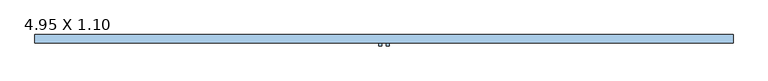
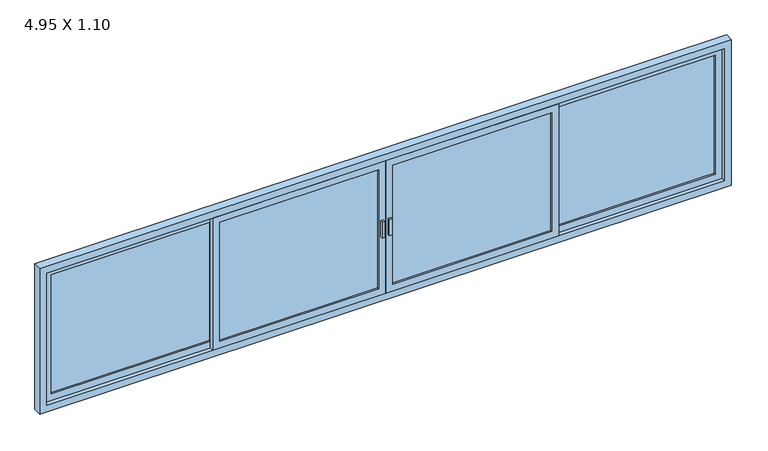
"""IFC4 building model written with IfcOpenShell, lengths in millimetres: window geometry, .CC_ND 300_JANELA_4 FOLHAS DE CORRER_VIDRO : 4.95 X 1.10."""

import ifcopenshell
import ifcopenshell.guid

model = None  # the IFC model being written
_history = None  # IfcOwnerHistory: only IFC2X3 demands one
_inside = {}  # id of a spatial element -> (the spatial element, [elements in it])
_under = {}  # id of a project, library or spatial element -> (it, [spatial elements below it])
_declared = {}  # id of a project -> (the project, [libraries it declares])
_typed = {}  # id of a type object -> (the type object, [elements of that type])
_made_of = {}  # id of a material, layer set ... -> (it, [elements and type objects made of it])


def new_model(schema):
    """Start an empty IFC model of exactly this schema.

    Asked for "IFC4X3", IfcOpenShell would pick the latest addendum, in which some entities
    have other attributes; the version numbers below select the first issue.
    IFC2X3 requires an IfcOwnerHistory on every rooted entity: one is made here for all.
    """
    global model, _history
    if schema == "IFC4X3":
        model = ifcopenshell.file(schema_version=(4, 3, 0, 0))
    else:
        model = ifcopenshell.file(schema=schema)
    _inside.clear()
    _under.clear()
    _declared.clear()
    _typed.clear()
    _made_of.clear()
    _history = None
    if model.schema == "IFC2X3":
        org = make("IfcOrganization", Name="unknown")
        user = make(
            "IfcPersonAndOrganization",
            ThePerson=make("IfcPerson", FamilyName="unknown"),
            TheOrganization=org,
        )
        app = make(
            "IfcApplication",
            ApplicationDeveloper=org,
            Version="unknown",
            ApplicationFullName="unknown",
            ApplicationIdentifier="unknown",
        )
        _history = make(
            "IfcOwnerHistory",
            OwningUser=user,
            OwningApplication=app,
            ChangeAction="ADDED",
            CreationDate=0,
        )
    return model


def make(cls, **values):
    """One entity of the class cls with the attributes given. An attribute that is None is left unset."""
    return model.create_entity(
        cls, **{name: value for name, value in values.items() if value is not None}
    )


def rooted(cls, **values):
    """An entity with a GlobalId (a new one), such as an element, a storey or a relation."""
    return make(cls, GlobalId=ifcopenshell.guid.new(), OwnerHistory=_history, **values)


def si_unit(unit_type, name, prefix=None):
    """IfcSIUnit, for example si_unit("LENGTHUNIT", "METRE", prefix="MILLI")."""
    return make("IfcSIUnit", UnitType=unit_type, Prefix=prefix, Name=name)


def assignment(units):
    """IfcUnitAssignment: the units of a project."""
    return None if units is None else make("IfcUnitAssignment", Units=units)


def point(xyz):
    """IfcCartesianPoint."""
    return None if xyz is None else make("IfcCartesianPoint", Coordinates=xyz)


def direction(xyz):
    """IfcDirection."""
    return None if xyz is None else make("IfcDirection", DirectionRatios=xyz)


def frame(location, z_axis=None, x_axis=None):
    """IfcAxis2Placement3D, a coordinate frame: its origin and axes. An axis left out is left unset."""
    return make(
        "IfcAxis2Placement3D",
        Location=point(location),
        Axis=direction(z_axis),
        RefDirection=direction(x_axis),
    )


def origin():
    """The frame at (0, 0, 0) with its axes left unset."""
    return frame((0.0, 0.0, 0.0))


def place(relative_to, where):
    """IfcLocalPlacement: puts the frame where relative to a parent placement (None: the world)."""
    return make(
        "IfcLocalPlacement", PlacementRelTo=relative_to, RelativePlacement=where
    )


def context(
    kind, dimensions, precision=None, world=None, true_north=None, identifier=None
):
    """IfcGeometricRepresentationContext, for example the 3D "Model" context."""
    return make(
        "IfcGeometricRepresentationContext",
        ContextIdentifier=identifier,
        ContextType=kind,
        CoordinateSpaceDimension=dimensions,
        Precision=precision,
        WorldCoordinateSystem=world,
        TrueNorth=true_north,
    )


def project(units=None, contexts=None):
    """IfcProject with its units and contexts."""
    return rooted(
        "IfcProject",
        Name="project",
        RepresentationContexts=contexts,
        UnitsInContext=assignment(units),
    )


def spatial(cls, under=None, at=None, **own):
    """A site, building, storey or space (cls), placed at a placement, below another one or the project."""
    s = rooted(cls, ObjectPlacement=at, **own)
    if under is not None:
        _under.setdefault(under.id(), (under, []))[1].append(s)
    return s


def polyline(points):
    """IfcPolyline through the points."""
    return make("IfcPolyline", Points=[point(p) for p in points])


def outline(outer, holes=None, kind="AREA"):
    """IfcArbitraryClosedProfileDef: a profile drawn as a closed curve; with holes, ...WithVoids."""
    if holes is None:
        return make("IfcArbitraryClosedProfileDef", ProfileType=kind, OuterCurve=outer)
    return make(
        "IfcArbitraryProfileDefWithVoids",
        ProfileType=kind,
        OuterCurve=outer,
        InnerCurves=holes,
    )


def extrude(swept, where, along, depth):
    """IfcExtrudedAreaSolid: the profile swept, set in the frame where, extruded along a direction by depth."""
    return make(
        "IfcExtrudedAreaSolid",
        SweptArea=swept,
        Position=where,
        ExtrudedDirection=direction(along),
        Depth=depth,
    )


def shape(context_of_items, identifier, shape_type, items):
    """IfcShapeRepresentation: the items that make up one representation, for example the "Body"."""
    return make(
        "IfcShapeRepresentation",
        ContextOfItems=context_of_items,
        RepresentationIdentifier=identifier,
        RepresentationType=shape_type,
        Items=items,
    )


def source(mapping_origin, context_of_items, identifier, shape_type, items):
    """IfcRepresentationMap: a shape defined once, which mapped items show again and again."""
    return make(
        "IfcRepresentationMap",
        MappingOrigin=mapping_origin,
        MappedRepresentation=shape(context_of_items, identifier, shape_type, items),
    )


def transform(
    local_origin,
    x_axis=None,
    y_axis=None,
    z_axis=None,
    scale=None,
    scale2=None,
    scale3=None,
    uniform=True,
):
    """IfcCartesianTransformationOperator3D, or its non-uniform kind. x_axis, y_axis, z_axis: its Axis1, 2, 3."""
    if uniform:
        return make(
            "IfcCartesianTransformationOperator3D",
            Axis1=direction(x_axis),
            Axis2=direction(y_axis),
            LocalOrigin=point(local_origin),
            Scale=scale,
            Axis3=direction(z_axis),
        )
    return make(
        "IfcCartesianTransformationOperator3DnonUniform",
        Axis1=direction(x_axis),
        Axis2=direction(y_axis),
        LocalOrigin=point(local_origin),
        Scale=scale,
        Axis3=direction(z_axis),
        Scale2=scale2,
        Scale3=scale3,
    )


def mapped(mapping_source, mapping_target):
    """IfcMappedItem: shows the shape of a source again, moved by a transform."""
    return make(
        "IfcMappedItem", MappingSource=mapping_source, MappingTarget=mapping_target
    )


def made_of(thing, what):
    """Note that an element or type object is made of a material, layer set ...; save() writes the relation."""
    if what is not None:
        _made_of.setdefault(what.id(), (what, []))[1].append(thing)
    return thing


def element(
    cls,
    number,
    at=None,
    inside=None,
    cuts=None,
    type_object=None,
    material=None,
    context=None,
    identifier="Body",
    shape_type=None,
    held_by="IfcProductDefinitionShape",
    body=None,
    shapes=None,
    **own,
):
    """One element of the class cls, such as IfcWall. Its Tag is "e" and its number.

    at: its placement. inside: the storey or other place that contains it. cuts: it is an
    opening in that element (IfcRelVoidsElement). A single representation is given by context,
    identifier, shape_type and body (its items); several are given by shapes. held_by: the class
    of the entity that holds the representations. save() writes the other relations.
    """
    e = rooted(cls, Tag="e%d" % number, ObjectPlacement=at, **own)
    if body is not None:
        shapes = [shape(context, identifier, shape_type, body)]
    if shapes is not None:
        e.Representation = make(held_by, Representations=shapes)
    if inside is not None:
        _inside.setdefault(inside.id(), (inside, []))[1].append(e)
    if cuts is not None:
        rooted(
            "IfcRelVoidsElement", RelatingBuildingElement=cuts, RelatedOpeningElement=e
        )
    if type_object is not None:
        _typed.setdefault(type_object.id(), (type_object, []))[1].append(e)
    return made_of(e, material)


def aggregate(whole, parts):
    """IfcRelAggregates: a whole, such as a stair, and the parts it consists of."""
    return rooted("IfcRelAggregates", RelatingObject=whole, RelatedObjects=parts)


def save(model, path):
    """Write the relations noted so far, then the file.

    IfcRelAggregates (storeys below a building ...), IfcRelContainedInSpatialStructure (elements
    in a storey), IfcRelDefinesByType, IfcRelAssociatesMaterial and IfcRelDeclares: one each for
    every whole, place, type object, material and project.
    """
    for whole, parts in _under.values():
        aggregate(whole, parts)
    for where, things in _inside.values():
        rooted(
            "IfcRelContainedInSpatialStructure",
            RelatedElements=things,
            RelatingStructure=where,
        )
    for kind, things in _typed.values():
        rooted("IfcRelDefinesByType", RelatedObjects=things, RelatingType=kind)
    for what, things in _made_of.values():
        rooted("IfcRelAssociatesMaterial", RelatedObjects=things, RelatingMaterial=what)
    for by, libraries in _declared.values():
        rooted("IfcRelDeclares", RelatingContext=by, RelatedDefinitions=libraries)
    model.write(path)


def window_4_95_x_1_10_4a8d5465(model_context):
    return source(origin(), model_context, "Body", "SweptSolid", [
        extrude(outline(polyline([(-50.0, -12.5), (-50.0, -17.5), (-1187.5, -17.5), (-1187.5, -12.5), (-50.0, -12.5)])), frame((0.0, 0.0, 1100.0), z_axis=(0.0, 0.0, 1.0), x_axis=(1.0, 0.0, 0.0)), (0.0, 0.0, 1.0), 900.0),
        extrude(outline(polyline([(2050.0, 0.0), (2050.0, -1237.5), (1050.0, -1237.5), (1050.0, 0.0), (2050.0, 0.0)]), holes=[polyline([(2000.0, -50.0), (1100.0, -50.0), (1100.0, -1187.5), (2000.0, -1187.5), (2000.0, -50.0)])]), frame((0.0, -30.0, 0.0), z_axis=(0.0, 1.0, 0.0), x_axis=(0.0, 0.0, 1.0)), (0.0, 0.0, 1.0), 30.0),
        extrude(outline(polyline([(-1237.5, 17.5), (-1237.5, 12.5), (-2375.0, 12.5), (-2375.0, 17.5), (-1237.5, 17.5)])), frame((0.0, 0.0, 1100.0), z_axis=(0.0, 0.0, 1.0), x_axis=(1.0, 0.0, 0.0)), (0.0, 0.0, 1.0), 900.0),
        extrude(outline(polyline([(2050.0, -1187.5), (2050.0, -2425.0), (1050.0, -2425.0), (1050.0, -1187.5), (2050.0, -1187.5)]), holes=[polyline([(2000.0, -1237.5), (1100.0, -1237.5), (1100.0, -2375.0), (2000.0, -2375.0), (2000.0, -1237.5)])]), frame((0.0, 0.0, 0.0), z_axis=(0.0, 1.0, 0.0), x_axis=(0.0, 0.0, 1.0)), (0.0, 0.0, 1.0), 30.0),
        extrude(outline(polyline([(2375.0, 17.5), (2375.0, 12.5), (1237.5, 12.5), (1237.5, 17.5), (2375.0, 17.5)])), frame((0.0, 0.0, 1100.0), z_axis=(0.0, 0.0, 1.0), x_axis=(1.0, 0.0, 0.0)), (0.0, 0.0, 1.0), 900.0),
        extrude(outline(polyline([(2050.0, 2425.0), (2050.0, 1187.5), (1050.0, 1187.5), (1050.0, 2425.0), (2050.0, 2425.0)]), holes=[polyline([(2000.0, 2375.0), (1100.0, 2375.0), (1100.0, 1237.5), (2000.0, 1237.5), (2000.0, 2375.0)])]), frame((0.0, 0.0, 0.0), z_axis=(0.0, 1.0, 0.0), x_axis=(0.0, 0.0, 1.0)), (0.0, 0.0, 1.0), 30.0),
        extrude(outline(polyline([(1187.5, -12.5), (1187.5, -17.5), (50.0, -17.5), (50.0, -12.5), (1187.5, -12.5)])), frame((0.0, 0.0, 1100.0), z_axis=(0.0, 0.0, 1.0), x_axis=(1.0, 0.0, 0.0)), (0.0, 0.0, 1.0), 900.0),
        extrude(outline(polyline([(2050.0, 1237.5), (2050.0, 0.0), (1050.0, 0.0), (1050.0, 1237.5), (2050.0, 1237.5)]), holes=[polyline([(2000.0, 1187.5), (1100.0, 1187.5), (1100.0, 50.0), (2000.0, 50.0), (2000.0, 1187.5)])]), frame((0.0, -30.0, 0.0), z_axis=(0.0, 1.0, 0.0), x_axis=(0.0, 0.0, 1.0)), (0.0, 0.0, 1.0), 30.0),
        extrude(outline(polyline([(1000.0, -2475.0), (1000.0, 2475.0), (2100.0, 2475.0), (2100.0, -2475.0), (1000.0, -2475.0)]), holes=[polyline([(2050.0, -2425.0), (2050.0, 2425.0), (1050.0, 2425.0), (1050.0, -2425.0), (2050.0, -2425.0)])]), frame((0.0, -30.0, 0.0), z_axis=(0.0, 1.0, 0.0), x_axis=(0.0, 0.0, 1.0)), (0.0, 0.0, 1.0), 60.0),
        extrude(outline(polyline([(-35.9492003, -30.0), (-15.9492003, -30.0), (-15.9492003, -50.0), (-35.9492003, -50.0), (-35.9492003, -30.0)])), frame((0.0, 0.0, 1490.0), z_axis=(0.0, 0.0, 1.0), x_axis=(1.0, 0.0, 0.0)), (0.0, 0.0, 1.0), 120.0),
        extrude(outline(polyline([(15.9492003, -30.0), (35.9492003, -30.0), (35.9492003, -50.0), (15.9492003, -50.0), (15.9492003, -30.0)])), frame((0.0, 0.0, 1490.0), z_axis=(0.0, 0.0, 1.0), x_axis=(1.0, 0.0, 0.0)), (0.0, 0.0, 1.0), 120.0),
    ])


if __name__ == "__main__":
    model = new_model("IFC4")
    model_context = context("Model", 3, world=origin())
    ifc_project = project(units=[si_unit("LENGTHUNIT", "METRE", prefix="MILLI")], contexts=[model_context])
    site = spatial("IfcSite", under=ifc_project)
    building = spatial("IfcBuilding", under=site)
    placement = place(None, origin())
    window_4_95_x_1_10_shape = window_4_95_x_1_10_4a8d5465(model_context)
    element("IfcWindow", 1, ObjectType=".CC_ND 300_JANELA_4 FOLHAS DE CORRER_VIDRO : 4.95 X 1.10", at=placement, inside=building, context=model_context, shape_type="MappedRepresentation", body=[
        mapped(window_4_95_x_1_10_shape, transform((0.0, 0.0, 0.0), x_axis=(1.0, 0.0, 0.0), y_axis=(0.0, 1.0, 0.0), z_axis=(0.0, 0.0, 1.0))),
    ])
    save(model, "model.ifc")

# Revit data of these elements
# Type ".CC_ND 300_JANELA_4 FOLHAS DE CORRER_VIDRO : 4.95 X 1.10"
#   Type Mark = "69"
#   Largura moldura = 0.06 m
#   Largura janela = 4.85 m
#   Largura esquadria = 0.05 m
#   Largura do painel = 1.2375 m
#   Largura da moldura do painel = 0.05 m
#   Espessura painel = 0.03 m
#   Espessura moldura = 0.03 m
#   Altura janela = 1.00 m
#   Height = 1.10 m
#   Altura-padrão do peitoril = 1.00 m
#   Width = 4.95 m
#   Puxadores [instance default] = yes
#   Moldura interna [instance default] = yes
#   Moldura externa [instance default] = yes
#   Tipo de vidro = .VIDRO GENÉRICO
#   Material puxadores = .ALUMÍNIO COM PINTURA ELETROSTÁTICA BRANCA
#   Material moldura = .ALUMÍNIO COM PINTURA ELETROSTÁTICA BRANCA
#   Material da esquadria = .ALUMÍNIO COM PINTURA ELETROSTÁTICA BRANCA
#   Wall Closure = (empty or 0)
# Element 1 (IfcWindow, ".CC_ND 300_JANELA_4 FOLHAS DE CORRER_VIDRO : 4.95 X 1.10")
#   Moldura interna = no
#   Moldura externa = no
#   Materials on its faces: ".ALUMÍNIO COM PINTURA ELETROSTÁTICA BRANCA", ".VIDRO GENÉRICO"
# Materials
#   ".VIDRO GENÉRICO": class ".CC_VIDRO", colour RGB 0 128 192, transparency 0.9, Description = "Vidro comum", Cost = 0
#   ".ALUMÍNIO COM PINTURA ELETROSTÁTICA BRANCA": class "CC_METAIS", colour RGB 241 241 241, transparency 0, Cost = 0
